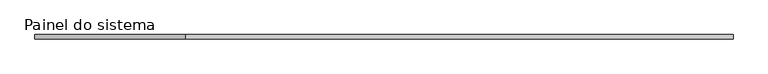
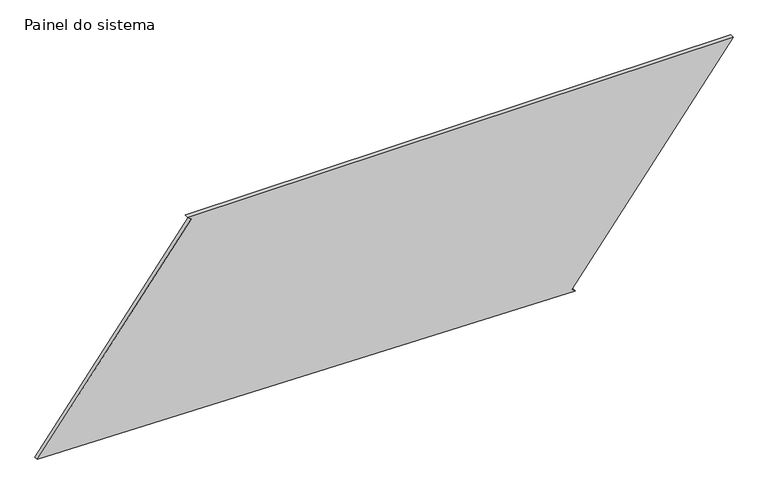
"""IFC4 building model written with IfcOpenShell, lengths in millimetres: plate geometry, Painel do sistema : Envidraçado."""

from ifc_helpers import new_model, si_unit, frame, origin, place, context, project, spatial, polyline, outline, extrude, source, transform, mapped, element, save


def painel_do_sistema_ec8ff91e(model_context):
    return source(origin(), model_context, "Body", "SweptSolid", [
        extrude(outline(polyline([(0.0, 1117.4678643), (15.2063352, 1097.6242917), (1254.6153953, 2047.396291), (1254.6153953, -1162.243673), (1239.4090602, -1142.4001005), (58.4303844, -2047.396291), (0.0, 1117.4678643)])), frame((0.0, 24.5, 0.0), z_axis=(0.0, 1.0, 0.0), x_axis=(0.0, 0.0, 1.0)), (0.0, 0.0, 1.0), 25.0),
    ])


if __name__ == "__main__":
    model = new_model("IFC4")
    model_context = context("Model", 3, world=origin())
    ifc_project = project(units=[si_unit("LENGTHUNIT", "METRE", prefix="MILLI")], contexts=[model_context])
    site = spatial("IfcSite", under=ifc_project)
    building = spatial("IfcBuilding", under=site)
    placement = place(None, origin())
    painel_do_sistema_shape = painel_do_sistema_ec8ff91e(model_context)
    element("IfcPlate", 1, ObjectType="Painel do sistema : Envidraçado", at=placement, inside=building, context=model_context, shape_type="MappedRepresentation", body=[
        mapped(painel_do_sistema_shape, transform((0.0, 0.0, 0.0), x_axis=(1.0, 0.0, 0.0), y_axis=(0.0, 1.0, 0.0), z_axis=(0.0, 0.0, 1.0))),
    ])
    save(model, "model.ifc")

# Revit data of these elements
# Type "Painel do sistema : Envidraçado"
#   Construction Type Id = "GSP4R"
#   Analytic Construction = "Vidraça única Pilkington 1/8 pol"
#   Visual Light Transmittance = 0.9
#   Solar Heat Gain Coefficient = 0.86
#   Heat Transfer Coefficient (U) = 6.7069 W/(m²·K)
# Element 1 (IfcPlate, "Painel do sistema : Envidraçado")
#   Materials on its faces: "Vidro"
# Materials
#   "Vidro": class "Vidro", colour RGB 0 128 192, transparency 0.9, Description = "Vidro de sílica", Cost = 0
